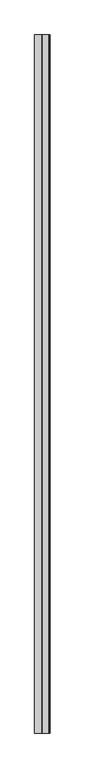
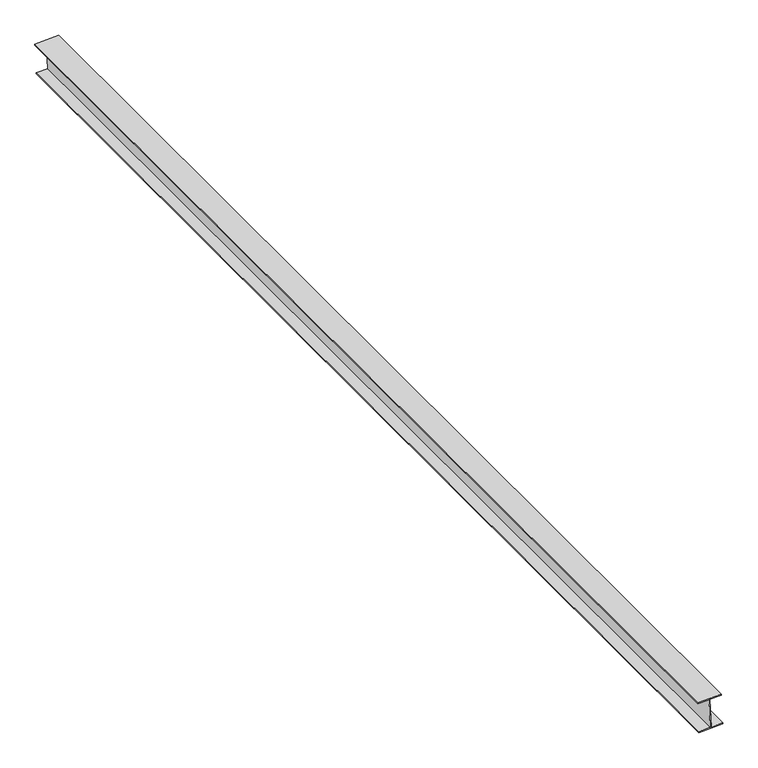
"""IFC4 building model written with IfcOpenShell, lengths in millimetres: proxy geometry, Generic Models 7:Generic Models 1:8:Generic Models 1:8 : Generic Models 7:Generic Models 1:337419:33 : Generic Models 7:Generic Models 1:8:Generic Models 1:8 : Generic Models 7:Generic Models 1:337419:315935."""

from ifc_helpers import new_model, si_unit, frame, origin, place, context, project, spatial, polyline, outline, extrude, source, transform, mapped, element, save


def generic_models_2c7ef85e(model_context):
    return source(origin(), model_context, "Body", "SweptSolid", [
        extrude(outline(polyline([(4024.8136317, 562936.6515986), (4027.7142797, 563009.6189671), (3838.3798209, 563017.1455182), (3835.4784389, 562944.1596862), (3828.6258513, 562944.4320949), (3834.6793776, 563096.7118205), (3841.5319652, 563096.4394118), (3838.621962, 563023.2367072), (4027.9564208, 563015.7101562), (4030.867158, 563088.9313242), (4037.7197456, 563088.6589155), (4031.6662193, 562936.3791899), (4024.8136317, 562936.6515986)])), frame((0.0, -578718.116384, 0.0), z_axis=(0.0, 1.0, 0.0), x_axis=(0.0, 0.0, 1.0)), (0.0, 0.0, 1.0), 7315.2),
    ])


if __name__ == "__main__":
    model = new_model("IFC4")
    model_context = context("Model", 3, world=origin())
    ifc_project = project(units=[si_unit("LENGTHUNIT", "METRE", prefix="MILLI")], contexts=[model_context])
    site = spatial("IfcSite", under=ifc_project)
    building = spatial("IfcBuilding", under=site)
    placement = place(None, origin())
    generic_models_shape = generic_models_2c7ef85e(model_context)
    element("IfcBuildingElementProxy", 1, Name="Generic Models 7:Generic Models 1:8:Generic Models 1:8 : Generic Models 7:Generic Models 1:337419:33 : Generic Models 7:Generic Models 1:8:Generic Models 1:8 : Generic Models 7:Generic Models 1:337419:315935", ObjectType="Generic Models 7:Generic Models 1:8:Generic Models 1:8 : Generic Models 7:Generic Models 1:337419:33 : Generic Models 7:Generic Models 1:8:Generic Models 1:8 : Generic Models 7:Generic Models 1:337419:315935", at=placement, inside=building, context=model_context, shape_type="MappedRepresentation", body=[
        mapped(generic_models_shape, transform((0.0, 0.0, 0.0), x_axis=(1.0, 0.0, 0.0), y_axis=(0.0, 1.0, 0.0), z_axis=(0.0, 0.0, 1.0))),
    ])
    save(model, "model.ifc")

# Revit data of these elements
# Type "Generic Models 7:Generic Models 1:8:Generic Models 1:8 : Generic Models 7:Generic Models 1:337419:33 : Generic Models 7:Generic Models 1:8:Generic Models 1:8 : Generic Models 7:Generic Models 1:337419:315935"
#   NameOverride = "Generic Models 7:Generic Models 1:8:Generic Models 1:8 : Generic Models 7:Generic Models 1:337419:315935"
#   ObjectTypeOverride = "Generic Models 1:8 : Generic Models 7:Generic Models 1:337419"
#   Reference = "Generic Models 1"
#   Tag = "315935"
# Element 1 (IfcBuildingElementProxy, "Generic Models 7:Generic Models 1:8:Generic Models 1:8 : Generic Models 7:Generic Models 1:337419:33 : Generic Models 7:Generic Models 1:8:Generic Models 1:8 : Generic Models 7:Generic Models 1:337419:315935")
#   Materials on its faces: "STRUCTURAL STEEL - SEE STRUCT. DWGS"
# Materials
#   "STRUCTURAL STEEL - SEE STRUCT. DWGS": class "Metal", colour RGB 189 187 185, transparency 0, Description = "Structural steel 50ksi", Cost = 0
